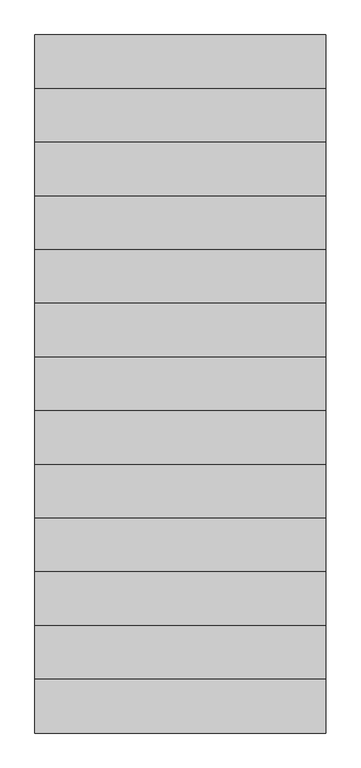
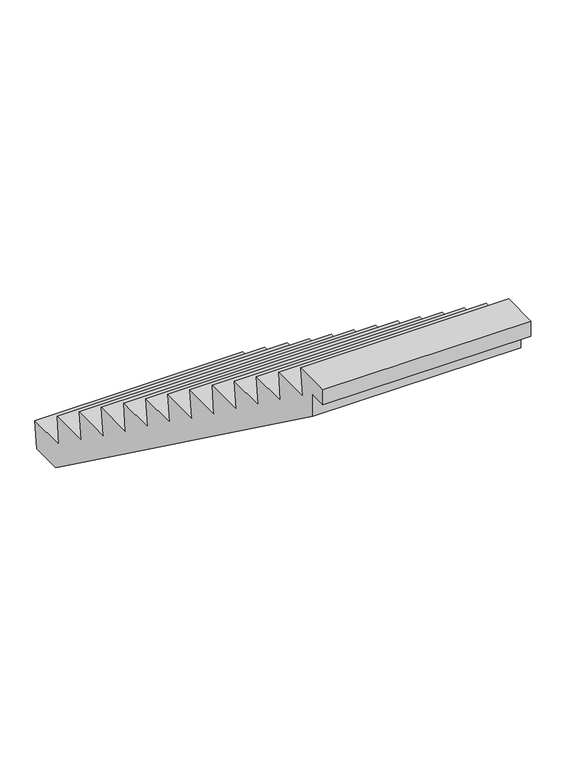
"""IFC4 building model written with IfcOpenShell, lengths in millimetres: proxy geometry, NLRS_24_GM_LB_rechte steektrap prefab-AV_gen_rsf : prefab trap_gen__aant=12 b=1200 a=220 o=172.7 zonder bomen."""

from ifc_helpers import new_model, si_unit, frame, origin, place, context, project, spatial, polyline, outline, extrude, source, transform, mapped, element, save


def generic_models_37fa75c9(model_context):
    return source(origin(), model_context, "Body", "SweptSolid", [
        extrude(outline(polyline([(-2880.0, 2270.0), (-2900.0, 2095.3846154), (-2640.0, 2095.3846154), (-2660.0, 1920.7692308), (-2400.0, 1920.7692308), (-2420.0, 1746.1538462), (-2160.0, 1746.1538462), (-2180.0, 1571.5384615), (-1920.0, 1571.5384615), (-1940.0, 1396.9230769), (-1680.0, 1396.9230769), (-1700.0, 1222.3076923), (-1440.0, 1222.3076923), (-1460.0, 1047.6923077), (-1200.0, 1047.6923077), (-1220.0, 873.0769231), (-960.0, 873.0769231), (-980.0, 698.4615385), (-720.0, 698.4615385), (-740.0, 523.8461538), (-480.0, 523.8461538), (-500.0, 349.2307692), (-240.0, 349.2307692), (-260.0, 174.6153846), (0.0, 174.6153846), (-20.0, 0.0), (-223.9686206, 0.0), (-3010.0, 2027.0164203), (-3010.0, 2170.0), (-3120.0, 2170.0), (-3120.0, 2270.0), (-2880.0, 2270.0)])), frame((-650.0, 0.0, 0.0), z_axis=(1.0, 0.0, 0.0), x_axis=(0.0, 1.0, 0.0)), (0.0, 0.0, 1.0), 1300.0),
    ])


if __name__ == "__main__":
    model = new_model("IFC4")
    model_context = context("Model", 3, world=origin())
    ifc_project = project(units=[si_unit("LENGTHUNIT", "METRE", prefix="MILLI")], contexts=[model_context])
    site = spatial("IfcSite", under=ifc_project)
    building = spatial("IfcBuilding", under=site)
    placement = place(None, origin())
    generic_models_shape = generic_models_37fa75c9(model_context)
    element("IfcBuildingElementProxy", 1, Name="NLRS_24_GM_LB_rechte steektrap prefab-AV_gen_rsf : prefab trap_gen__aant=12 b=1200 a=220 o=172.7 zonder bomen", ObjectType="NLRS_24_GM_LB_rechte steektrap prefab-AV_gen_rsf : prefab trap_gen__aant=12 b=1200 a=220 o=172.7 zonder bomen", at=placement, inside=building, context=model_context, shape_type="MappedRepresentation", body=[
        mapped(generic_models_shape, transform((0.0, 0.0, 0.0), x_axis=(1.0, 0.0, 0.0), y_axis=(0.0, 1.0, 0.0), z_axis=(0.0, 0.0, 1.0))),
    ])
    save(model, "model.ifc")

# Revit data of these elements
# Type "NLRS_24_GM_LB_rechte steektrap prefab-AV_gen_rsf : prefab trap_gen__aant=12 b=1200 a=220 o=172.7 zonder bomen"
#   Export Type to IFC As = "IfcStair"
#   Type IfcGUID = "2CEqVLPNH8KRN7ghwV3ZFx"
#   Type Comments = " "
#   Model = " "
#   Manufacturer = " "
#   Keynote = " "
#   Description = "rechte steektrap prefab\r\naant=11 b=1200 a=220 o=181,8\r\nzonder bomen"
#   Assembly Code = "24.11"
#   Aantrede onder = 240 mm
#   Width = 1300 mm
#   Wel diepte = 20 mm
#   Trapboom breedte = 0 mm
#   Thickness = 120 mm
#   Optrede onderste trede = 150 mm
#   NLRS_C_lengte = 2880 mm
#   Length = 3360 mm
#   Hoogte oplegnok onder = 100 mm
#   Hoogte oplegnok boven = 100 mm
#   Height = 2270 mm
#   Breedte oplegnok boven = 110 mm
#   BottomCalc = 150 mm
#   Actual Tread Depth = 240 mm
#   Actual Riser Height = 174.615 mm
#   Actual Number of Tread = 12
#   Actual Number of Risers = 13
#   Aantrede boven = 240 mm
#   Aantal treden max dertig = 13
#   Trapboom = no
#   Oplegnok onder = no
#   NLRS_C_materiaal = NLRS_f2_beton prefab_gen_rsf
#   Default Elevation = 0
# Element 1 (IfcBuildingElementProxy, "NLRS_24_GM_LB_rechte steektrap prefab-AV_gen_rsf : prefab trap_gen__aant=12 b=1200 a=220 o=172.7 zonder bomen")
#   Materials on its faces: "NLRS_f2_beton prefab_gen_rsf"
# Materials
#   "NLRS_f2_beton prefab_gen_rsf": class "F - Niet gebakken kunststeen", colour RGB 129 133 118, transparency 0, Keynote = "f2", Manufacturer = "Revit Standards Foundation", URL = "www.revitstandards.org", Description = "beton prefab", Cost = 0
